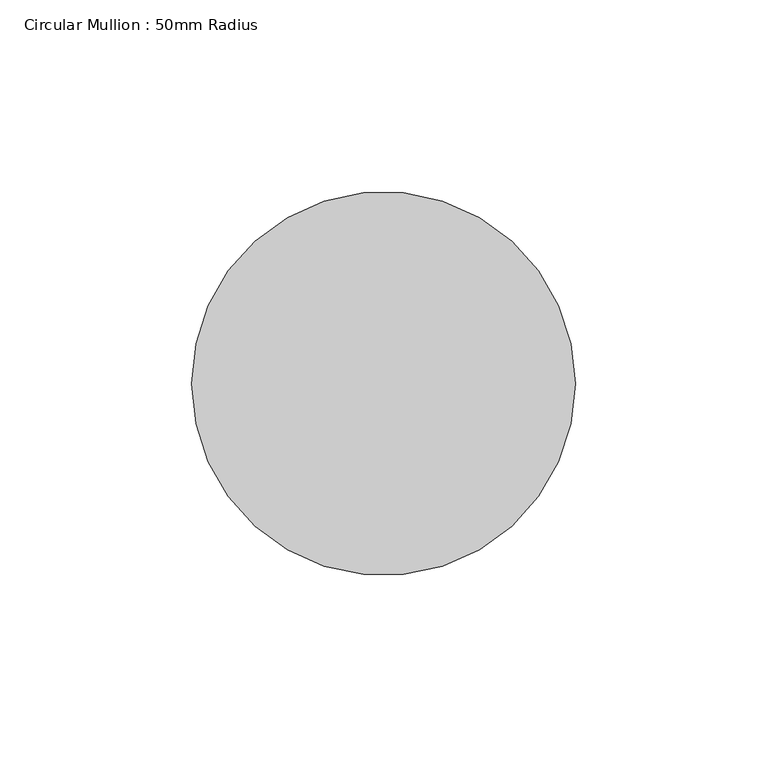
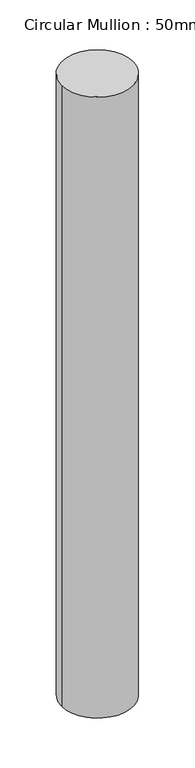
"""IFC4 building model written with IfcOpenShell, lengths in millimetres: member geometry, Circular Mullion : 50mm Radius."""

from ifc_helpers import new_model, si_unit, point, frame, origin, origin_2d, place, context, project, spatial, circle_curve, trimmed, segment, composite_curve, outline, extrude, source, transform, mapped, element, save


def circular_mullion_50mm_radius_4f1adb08(model_context):
    return source(origin(), model_context, "Body", "SweptSolid", [
        extrude(outline(composite_curve([segment(trimmed(circle_curve(origin_2d(), 50.0), [point((50.0, 0.0))], [point((-50.0, 0.0))], False, "CARTESIAN"), True, "CONTINUOUS"), segment(trimmed(circle_curve(origin_2d(), 50.0), [point((-50.0, 0.0))], [point((50.0, 0.0))], False, "CARTESIAN"), True, "CONTINUOUS")], self_intersect=False)), frame((0.0, 0.0, -920.8544168), z_axis=(0.0, 0.0, 1.0), x_axis=(1.0, 0.0, 0.0)), (0.0, 0.0, 1.0), 920.8544168),
    ])


if __name__ == "__main__":
    model = new_model("IFC4")
    model_context = context("Model", 3, world=origin())
    ifc_project = project(units=[si_unit("LENGTHUNIT", "METRE", prefix="MILLI")], contexts=[model_context])
    site = spatial("IfcSite", under=ifc_project)
    building = spatial("IfcBuilding", under=site)
    placement = place(None, origin())
    circular_mullion_50mm_radius_shape = circular_mullion_50mm_radius_4f1adb08(model_context)
    element("IfcMember", 1, ObjectType="Circular Mullion : 50mm Radius", at=placement, inside=building, context=model_context, shape_type="MappedRepresentation", body=[
        mapped(circular_mullion_50mm_radius_shape, transform((0.0, 0.0, 0.0), x_axis=(1.0, 0.0, 0.0), y_axis=(0.0, 1.0, 0.0), z_axis=(0.0, 0.0, 1.0))),
    ])
    save(model, "model.ifc")

# Revit data of these elements
# Type "Circular Mullion : 50mm Radius"
#   built-in parameter 1007350 = 0.164042 (stored number, unit not read)
# Element 1 (IfcMember, "Circular Mullion : 50mm Radius")
#   Materials on its faces: "Aluminium"
# Materials
#   "Aluminium": class "Metal", colour RGB 247 247 247, transparency 0, Description = "Aluminium 6061", Cost = 0
